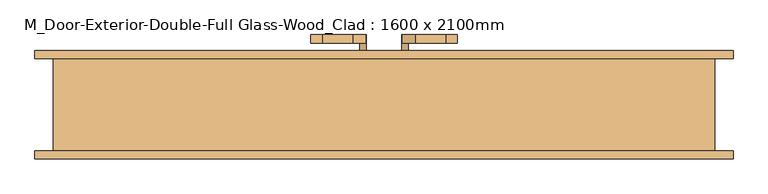
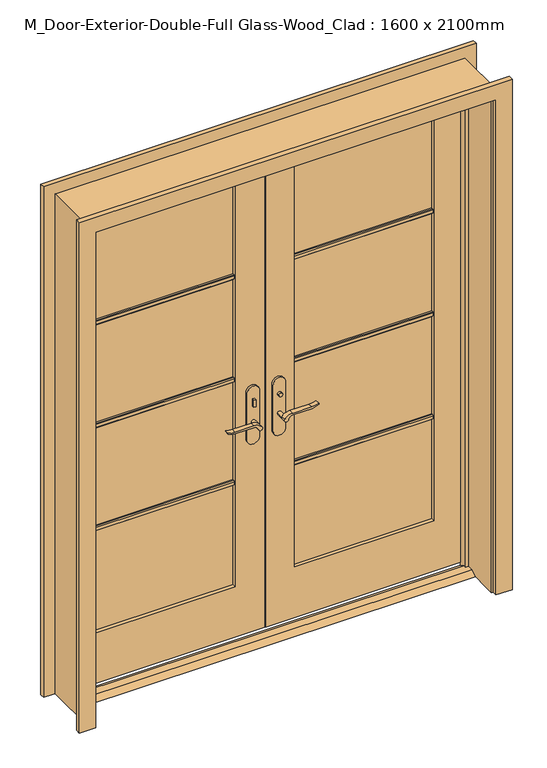
"""IFC4 building model written with IfcOpenShell, lengths in millimetres: door geometry, M_Door-Exterior-Double-Full Glass-Wood_Clad : 1600 x 2100mm."""

import ifcopenshell
import ifcopenshell.guid

model = None  # the IFC model being written
_history = None  # IfcOwnerHistory: only IFC2X3 demands one
_inside = {}  # id of a spatial element -> (the spatial element, [elements in it])
_under = {}  # id of a project, library or spatial element -> (it, [spatial elements below it])
_declared = {}  # id of a project -> (the project, [libraries it declares])
_typed = {}  # id of a type object -> (the type object, [elements of that type])
_made_of = {}  # id of a material, layer set ... -> (it, [elements and type objects made of it])


def new_model(schema):
    """Start an empty IFC model of exactly this schema.

    Asked for "IFC4X3", IfcOpenShell would pick the latest addendum, in which some entities
    have other attributes; the version numbers below select the first issue.
    IFC2X3 requires an IfcOwnerHistory on every rooted entity: one is made here for all.
    """
    global model, _history
    if schema == "IFC4X3":
        model = ifcopenshell.file(schema_version=(4, 3, 0, 0))
    else:
        model = ifcopenshell.file(schema=schema)
    _inside.clear()
    _under.clear()
    _declared.clear()
    _typed.clear()
    _made_of.clear()
    _history = None
    if model.schema == "IFC2X3":
        org = make("IfcOrganization", Name="unknown")
        user = make(
            "IfcPersonAndOrganization",
            ThePerson=make("IfcPerson", FamilyName="unknown"),
            TheOrganization=org,
        )
        app = make(
            "IfcApplication",
            ApplicationDeveloper=org,
            Version="unknown",
            ApplicationFullName="unknown",
            ApplicationIdentifier="unknown",
        )
        _history = make(
            "IfcOwnerHistory",
            OwningUser=user,
            OwningApplication=app,
            ChangeAction="ADDED",
            CreationDate=0,
        )
    return model


def make(cls, **values):
    """One entity of the class cls with the attributes given. An attribute that is None is left unset."""
    return model.create_entity(
        cls, **{name: value for name, value in values.items() if value is not None}
    )


def rooted(cls, **values):
    """An entity with a GlobalId (a new one), such as an element, a storey or a relation."""
    return make(cls, GlobalId=ifcopenshell.guid.new(), OwnerHistory=_history, **values)


def si_unit(unit_type, name, prefix=None):
    """IfcSIUnit, for example si_unit("LENGTHUNIT", "METRE", prefix="MILLI")."""
    return make("IfcSIUnit", UnitType=unit_type, Prefix=prefix, Name=name)


def assignment(units):
    """IfcUnitAssignment: the units of a project."""
    return None if units is None else make("IfcUnitAssignment", Units=units)


def point(xyz):
    """IfcCartesianPoint."""
    return None if xyz is None else make("IfcCartesianPoint", Coordinates=xyz)


def direction(xyz):
    """IfcDirection."""
    return None if xyz is None else make("IfcDirection", DirectionRatios=xyz)


def frame(location, z_axis=None, x_axis=None):
    """IfcAxis2Placement3D, a coordinate frame: its origin and axes. An axis left out is left unset."""
    return make(
        "IfcAxis2Placement3D",
        Location=point(location),
        Axis=direction(z_axis),
        RefDirection=direction(x_axis),
    )


def frame_2d(location, x_axis=None):
    """IfcAxis2Placement2D, a coordinate frame in the plane: its origin and x axis."""
    return make(
        "IfcAxis2Placement2D", Location=point(location), RefDirection=direction(x_axis)
    )


def origin():
    """The frame at (0, 0, 0) with its axes left unset."""
    return frame((0.0, 0.0, 0.0))


def place(relative_to, where):
    """IfcLocalPlacement: puts the frame where relative to a parent placement (None: the world)."""
    return make(
        "IfcLocalPlacement", PlacementRelTo=relative_to, RelativePlacement=where
    )


def context(
    kind, dimensions, precision=None, world=None, true_north=None, identifier=None
):
    """IfcGeometricRepresentationContext, for example the 3D "Model" context."""
    return make(
        "IfcGeometricRepresentationContext",
        ContextIdentifier=identifier,
        ContextType=kind,
        CoordinateSpaceDimension=dimensions,
        Precision=precision,
        WorldCoordinateSystem=world,
        TrueNorth=true_north,
    )


def project(units=None, contexts=None):
    """IfcProject with its units and contexts."""
    return rooted(
        "IfcProject",
        Name="project",
        RepresentationContexts=contexts,
        UnitsInContext=assignment(units),
    )


def spatial(cls, under=None, at=None, **own):
    """A site, building, storey or space (cls), placed at a placement, below another one or the project."""
    s = rooted(cls, ObjectPlacement=at, **own)
    if under is not None:
        _under.setdefault(under.id(), (under, []))[1].append(s)
    return s


def polyline(points):
    """IfcPolyline through the points."""
    return make("IfcPolyline", Points=[point(p) for p in points])


def circle_curve(where, radius):
    """IfcCircle in the frame where."""
    return make("IfcCircle", Position=where, Radius=radius)


def trimmed(basis, trim1, trim2, sense, master):
    """IfcTrimmedCurve: the piece of a basis curve between two trims."""
    return make(
        "IfcTrimmedCurve",
        BasisCurve=basis,
        Trim1=trim1,
        Trim2=trim2,
        SenseAgreement=sense,
        MasterRepresentation=master,
    )


def segment(curve, same_sense, transition):
    """IfcCompositeCurveSegment."""
    return make(
        "IfcCompositeCurveSegment",
        Transition=transition,
        SameSense=same_sense,
        ParentCurve=curve,
    )


def composite_curve(segments, self_intersect=None):
    """IfcCompositeCurve: segments joined end to end."""
    return make("IfcCompositeCurve", Segments=segments, SelfIntersect=self_intersect)


def outline(outer, holes=None, kind="AREA"):
    """IfcArbitraryClosedProfileDef: a profile drawn as a closed curve; with holes, ...WithVoids."""
    if holes is None:
        return make("IfcArbitraryClosedProfileDef", ProfileType=kind, OuterCurve=outer)
    return make(
        "IfcArbitraryProfileDefWithVoids",
        ProfileType=kind,
        OuterCurve=outer,
        InnerCurves=holes,
    )


def extrude(swept, where, along, depth):
    """IfcExtrudedAreaSolid: the profile swept, set in the frame where, extruded along a direction by depth."""
    return make(
        "IfcExtrudedAreaSolid",
        SweptArea=swept,
        Position=where,
        ExtrudedDirection=direction(along),
        Depth=depth,
    )


def faces_of(points, faces, orient=None, outer=None):
    """IfcFace entities. A face is a list of loops; a loop is a list of indices into points, from 0.

    orient and outer hold one flag for each loop. By default every Orientation is true, the
    first loop of a face is its IfcFaceOuterBound and the others are IfcFaceBound.
    """
    made = []
    for i, loops in enumerate(faces):
        bounds = []
        for j, loop in enumerate(loops):
            is_outer = j == 0 if outer is None else outer[i][j]
            bounds.append(
                make(
                    "IfcFaceOuterBound" if is_outer else "IfcFaceBound",
                    Bound=make("IfcPolyLoop", Polygon=[points[k] for k in loop]),
                    Orientation=True if orient is None else orient[i][j],
                )
            )
        made.append(make("IfcFace", Bounds=bounds))
    return made


def faceted_brep(points, faces, orient=None, outer=None, voids=None):
    """IfcFacetedBrep: a solid bounded by flat faces; with voids (closed shells), ...WithVoids."""
    shared = [point(p) for p in points]
    hull = make("IfcClosedShell", CfsFaces=faces_of(shared, faces, orient, outer))
    if voids is None:
        return make("IfcFacetedBrep", Outer=hull)
    return make(
        "IfcFacetedBrepWithVoids",
        Outer=hull,
        Voids=[
            make(cls, CfsFaces=faces_of(shared, fs, o, b)) for cls, fs, o, b in voids
        ],
    )


def shape(context_of_items, identifier, shape_type, items):
    """IfcShapeRepresentation: the items that make up one representation, for example the "Body"."""
    return make(
        "IfcShapeRepresentation",
        ContextOfItems=context_of_items,
        RepresentationIdentifier=identifier,
        RepresentationType=shape_type,
        Items=items,
    )


def source(mapping_origin, context_of_items, identifier, shape_type, items):
    """IfcRepresentationMap: a shape defined once, which mapped items show again and again."""
    return make(
        "IfcRepresentationMap",
        MappingOrigin=mapping_origin,
        MappedRepresentation=shape(context_of_items, identifier, shape_type, items),
    )


def transform(
    local_origin,
    x_axis=None,
    y_axis=None,
    z_axis=None,
    scale=None,
    scale2=None,
    scale3=None,
    uniform=True,
):
    """IfcCartesianTransformationOperator3D, or its non-uniform kind. x_axis, y_axis, z_axis: its Axis1, 2, 3."""
    if uniform:
        return make(
            "IfcCartesianTransformationOperator3D",
            Axis1=direction(x_axis),
            Axis2=direction(y_axis),
            LocalOrigin=point(local_origin),
            Scale=scale,
            Axis3=direction(z_axis),
        )
    return make(
        "IfcCartesianTransformationOperator3DnonUniform",
        Axis1=direction(x_axis),
        Axis2=direction(y_axis),
        LocalOrigin=point(local_origin),
        Scale=scale,
        Axis3=direction(z_axis),
        Scale2=scale2,
        Scale3=scale3,
    )


def mapped(mapping_source, mapping_target):
    """IfcMappedItem: shows the shape of a source again, moved by a transform."""
    return make(
        "IfcMappedItem", MappingSource=mapping_source, MappingTarget=mapping_target
    )


def made_of(thing, what):
    """Note that an element or type object is made of a material, layer set ...; save() writes the relation."""
    if what is not None:
        _made_of.setdefault(what.id(), (what, []))[1].append(thing)
    return thing


def element(
    cls,
    number,
    at=None,
    inside=None,
    cuts=None,
    type_object=None,
    material=None,
    context=None,
    identifier="Body",
    shape_type=None,
    held_by="IfcProductDefinitionShape",
    body=None,
    shapes=None,
    **own,
):
    """One element of the class cls, such as IfcWall. Its Tag is "e" and its number.

    at: its placement. inside: the storey or other place that contains it. cuts: it is an
    opening in that element (IfcRelVoidsElement). A single representation is given by context,
    identifier, shape_type and body (its items); several are given by shapes. held_by: the class
    of the entity that holds the representations. save() writes the other relations.
    """
    e = rooted(cls, Tag="e%d" % number, ObjectPlacement=at, **own)
    if body is not None:
        shapes = [shape(context, identifier, shape_type, body)]
    if shapes is not None:
        e.Representation = make(held_by, Representations=shapes)
    if inside is not None:
        _inside.setdefault(inside.id(), (inside, []))[1].append(e)
    if cuts is not None:
        rooted(
            "IfcRelVoidsElement", RelatingBuildingElement=cuts, RelatedOpeningElement=e
        )
    if type_object is not None:
        _typed.setdefault(type_object.id(), (type_object, []))[1].append(e)
    return made_of(e, material)


def aggregate(whole, parts):
    """IfcRelAggregates: a whole, such as a stair, and the parts it consists of."""
    return rooted("IfcRelAggregates", RelatingObject=whole, RelatedObjects=parts)


def save(model, path):
    """Write the relations noted so far, then the file.

    IfcRelAggregates (storeys below a building ...), IfcRelContainedInSpatialStructure (elements
    in a storey), IfcRelDefinesByType, IfcRelAssociatesMaterial and IfcRelDeclares: one each for
    every whole, place, type object, material and project.
    """
    for whole, parts in _under.values():
        aggregate(whole, parts)
    for where, things in _inside.values():
        rooted(
            "IfcRelContainedInSpatialStructure",
            RelatedElements=things,
            RelatingStructure=where,
        )
    for kind, things in _typed.values():
        rooted("IfcRelDefinesByType", RelatedObjects=things, RelatingType=kind)
    for what, things in _made_of.values():
        rooted("IfcRelAssociatesMaterial", RelatedObjects=things, RelatingMaterial=what)
    for by, libraries in _declared.values():
        rooted("IfcRelDeclares", RelatingContext=by, RelatedDefinitions=libraries)
    model.write(path)


def m_door_exterior_double_full_glass_wood_clad_1600_x_2100mm_56e3e291(model_context):
    return source(origin(), model_context, "Body", "SolidModel", [
        extrude(outline(polyline([(18.975, 15.0), (53.975, 15.0), (79.375, 0.0), (-6.425, 0.0), (18.975, 15.0)])), frame((-800.0, 0.0, 0.0), z_axis=(1.0, 0.0, 0.0), x_axis=(0.0, 1.0, 0.0)), (0.0, 0.0, 1.0), 1600.0),
        extrude(outline(polyline([(-47.4019111, 56.825), (-57.4019111, 56.825), (-57.4019111, 66.825), (-47.4019111, 66.825), (-47.4019111, 56.825)])), frame((0.0, 0.0, 981.9), z_axis=(0.0, 0.0, 1.0), x_axis=(1.0, 0.0, 0.0)), (0.0, 0.0, 1.0), 30.0),
        extrude(outline(composite_curve([segment(trimmed(circle_curve(frame_2d((996.9, -52.4019111)), 8.0), [point((996.9, -60.4019111))], [point((996.9, -44.4019111))], False, "CARTESIAN"), True, "CONTINUOUS"), segment(trimmed(circle_curve(frame_2d((996.9, -52.4019111)), 8.0), [point((996.9, -44.4019111))], [point((996.9, -60.4019111))], False, "CARTESIAN"), True, "CONTINUOUS")], self_intersect=False)), frame((0.0, 121.825, 0.0), z_axis=(0.0, 1.0, 0.0), x_axis=(0.0, 0.0, 1.0)), (0.0, 0.0, 1.0), 10.0),
        extrude(outline(composite_curve([segment(trimmed(circle_curve(frame_2d((897.1555521, -76.0694241)), 37.2832219), [point((919.0523287, -45.8937749))], [point((934.4, -77.7693445))], False, "CARTESIAN"), True, "CONTINUOUS"), segment(polyline([(934.4, -77.7693445), (934.4, -154.045502)]), True, "CONTINUOUS"), segment(trimmed(circle_curve(frame_2d((1017.6850638, -153.9791202)), 83.2850902), [point((934.4, -154.045502))], [point((939.4, -182.4019111))], True, "CARTESIAN"), True, "CONTINUOUS"), segment(polyline([(939.4, -182.4019111), (936.6135558, -182.4019111)]), True, "CONTINUOUS"), segment(trimmed(circle_curve(frame_2d((986.6709207, -150.4622499)), 59.3791355), [point((936.6135558, -182.4019111))], [point((927.4, -154.045502))], False, "CARTESIAN"), True, "CONTINUOUS"), segment(polyline([(927.4, -154.045502), (927.4, -77.7881013)]), True, "CONTINUOUS"), segment(trimmed(circle_curve(frame_2d((909.2738613, -77.7881013)), 18.1261387), [point((927.4, -77.7881013))], [point((914.4, -60.4019111))], True, "CARTESIAN"), True, "CONTINUOUS"), segment(trimmed(circle_curve(frame_2d((914.4, -52.4019111)), 8.0), [point((914.4, -60.4019111))], [point((919.0523287, -45.8937749))], False, "CARTESIAN"), True, "CONTINUOUS")], self_intersect=False)), frame((0.0, 16.825, 0.0), z_axis=(0.0, 1.0, 0.0), x_axis=(0.0, 0.0, 1.0)), (0.0, 0.0, 1.0), 20.0),
        extrude(outline(composite_curve([segment(trimmed(circle_curve(frame_2d((914.4, -52.4019111)), 8.0), [point((914.3999903, -60.4019111))], [point((919.0523287, -45.8937749))], False, "CARTESIAN"), True, "CONTINUOUS"), segment(trimmed(circle_curve(frame_2d((897.1555521, -76.0694241)), 37.2832219), [point((919.0523287, -45.8937749))], [point((934.4, -77.7693445))], False, "CARTESIAN"), True, "CONTINUOUS"), segment(polyline([(934.4, -77.7693445), (934.4, -154.045502)]), True, "CONTINUOUS"), segment(trimmed(circle_curve(frame_2d((1017.6850638, -153.9791202)), 83.2850902), [point((934.4, -154.045502))], [point((939.4, -182.4019111))], True, "CARTESIAN"), True, "CONTINUOUS"), segment(polyline([(939.4, -182.4019111), (936.6135558, -182.4019111)]), True, "CONTINUOUS"), segment(trimmed(circle_curve(frame_2d((986.6709207, -150.4622499)), 59.3791355), [point((936.6135558, -182.4019111))], [point((927.4, -154.045502))], False, "CARTESIAN"), True, "CONTINUOUS"), segment(polyline([(927.4, -154.045502), (927.4, -77.788099)]), True, "CONTINUOUS"), segment(trimmed(circle_curve(frame_2d((909.2738682, -77.788099)), 18.1261318), [point((927.4, -77.788099))], [point((914.3999903, -60.4019111))], True, "CARTESIAN"), True, "CONTINUOUS")], self_intersect=False)), frame((0.0, 151.825, 0.0), z_axis=(0.0, 1.0, 0.0), x_axis=(0.0, 0.0, 1.0)), (0.0, 0.0, 1.0), 20.0),
        extrude(outline(composite_curve([segment(trimmed(circle_curve(frame_2d((914.4, -52.4019111)), 8.0), [point((914.4, -60.4019111))], [point((914.4, -44.4019111))], False, "CARTESIAN"), True, "CONTINUOUS"), segment(trimmed(circle_curve(frame_2d((914.4, -52.4019111)), 8.0), [point((914.4, -44.4019111))], [point((914.4, -60.4019111))], False, "CARTESIAN"), True, "CONTINUOUS")], self_intersect=False)), frame((0.0, 36.825, 0.0), z_axis=(0.0, 1.0, 0.0), x_axis=(0.0, 0.0, 1.0)), (0.0, 0.0, 1.0), 30.0),
        extrude(outline(composite_curve([segment(trimmed(circle_curve(frame_2d((914.4, -52.4019111)), 8.0), [point((914.4, -60.4019111))], [point((914.4, -44.4019111))], False, "CARTESIAN"), True, "CONTINUOUS"), segment(trimmed(circle_curve(frame_2d((914.4, -52.4019111)), 8.0), [point((914.4, -44.4019111))], [point((914.4, -60.4019111))], False, "CARTESIAN"), True, "CONTINUOUS")], self_intersect=False)), frame((0.0, 121.825, 0.0), z_axis=(0.0, 1.0, 0.0), x_axis=(0.0, 0.0, 1.0)), (0.0, 0.0, 1.0), 30.0),
        extrude(outline(composite_curve([segment(polyline([(844.4, -27.4019111), (1039.4, -27.4019111)]), True, "CONTINUOUS"), segment(trimmed(circle_curve(frame_2d((1039.4, -52.4019111)), 25.0), [point((1039.4, -27.4019111))], [point((1039.4, -77.4019111))], False, "CARTESIAN"), True, "CONTINUOUS"), segment(polyline([(1039.4, -77.4019111), (844.4, -77.4019111)]), True, "CONTINUOUS"), segment(trimmed(circle_curve(frame_2d((844.4, -52.4019111)), 25.0), [point((844.4, -77.4019111))], [point((844.4, -27.4019111))], False, "CARTESIAN"), True, "CONTINUOUS")], self_intersect=False)), frame((0.0, 66.825, 0.0), z_axis=(0.0, 1.0, 0.0), x_axis=(0.0, 0.0, 1.0)), (0.0, 0.0, 1.0), 10.0),
        extrude(outline(composite_curve([segment(polyline([(844.4, -27.4019111), (1039.4, -27.4019111)]), True, "CONTINUOUS"), segment(trimmed(circle_curve(frame_2d((1039.4, -52.4019111)), 25.0), [point((1039.4, -27.4019111))], [point((1039.4, -77.4019111))], False, "CARTESIAN"), True, "CONTINUOUS"), segment(polyline([(1039.4, -77.4019111), (844.4, -77.4019111)]), True, "CONTINUOUS"), segment(trimmed(circle_curve(frame_2d((844.4, -52.4019111)), 25.0), [point((844.4, -77.4019111))], [point((844.4, -27.4019111))], False, "CARTESIAN"), True, "CONTINUOUS")], self_intersect=False)), frame((0.0, 111.825, 0.0), z_axis=(0.0, 1.0, 0.0), x_axis=(0.0, 0.0, 1.0)), (0.0, 0.0, 1.0), 10.0),
        extrude(outline(polyline([(47.3875, 131.825), (57.3875, 131.825), (57.3875, 121.825), (47.3875, 121.825), (47.3875, 131.825)])), frame((0.0, 0.0, 981.9), z_axis=(0.0, 0.0, 1.0), x_axis=(1.0, 0.0, 0.0)), (0.0, 0.0, 1.0), 30.0),
        extrude(outline(composite_curve([segment(trimmed(circle_curve(frame_2d((996.9, 52.3875)), 8.0), [point((996.9, 60.3875))], [point((996.9, 44.3875))], False, "CARTESIAN"), True, "CONTINUOUS"), segment(trimmed(circle_curve(frame_2d((996.9, 52.3875)), 8.0), [point((996.9, 44.3875))], [point((996.9, 60.3875))], False, "CARTESIAN"), True, "CONTINUOUS")], self_intersect=False)), frame((0.0, 56.825, 0.0), z_axis=(0.0, 1.0, 0.0), x_axis=(0.0, 0.0, 1.0)), (0.0, 0.0, 1.0), 10.0),
        extrude(outline(composite_curve([segment(trimmed(circle_curve(frame_2d((914.4, 52.3875)), 8.0), [point((919.0523287, 45.8793637))], [point((914.4, 60.3875))], False, "CARTESIAN"), True, "CONTINUOUS"), segment(trimmed(circle_curve(frame_2d((909.2738613, 77.7736901)), 18.1261387), [point((914.4, 60.3875))], [point((927.4, 77.7736901))], True, "CARTESIAN"), True, "CONTINUOUS"), segment(polyline([(927.4, 77.7736901), (927.4, 154.0310909)]), True, "CONTINUOUS"), segment(trimmed(circle_curve(frame_2d((986.6709207, 150.4478388)), 59.3791355), [point((927.4, 154.0310909))], [point((936.6135558, 182.3875))], False, "CARTESIAN"), True, "CONTINUOUS"), segment(polyline([(936.6135558, 182.3875), (939.4, 182.3875)]), True, "CONTINUOUS"), segment(trimmed(circle_curve(frame_2d((1017.6850638, 153.9647091)), 83.2850902), [point((939.4, 182.3875))], [point((934.4, 154.0310909))], True, "CARTESIAN"), True, "CONTINUOUS"), segment(polyline([(934.4, 154.0310909), (934.4, 77.7549333)]), True, "CONTINUOUS"), segment(trimmed(circle_curve(frame_2d((897.1555521, 76.0550129)), 37.2832219), [point((934.4, 77.7549333))], [point((919.0523287, 45.8793637))], False, "CARTESIAN"), True, "CONTINUOUS")], self_intersect=False)), frame((0.0, 151.825, 0.0), z_axis=(0.0, 1.0, 0.0), x_axis=(0.0, 0.0, 1.0)), (0.0, 0.0, 1.0), 20.0),
        extrude(outline(composite_curve([segment(trimmed(circle_curve(frame_2d((909.2738682, 77.7736878)), 18.1261318), [point((914.3999903, 60.3875))], [point((927.4, 77.7736878))], True, "CARTESIAN"), True, "CONTINUOUS"), segment(polyline([(927.4, 77.7736878), (927.4, 154.0310909)]), True, "CONTINUOUS"), segment(trimmed(circle_curve(frame_2d((986.6709207, 150.4478388)), 59.3791355), [point((927.4, 154.0310909))], [point((936.6135558, 182.3875))], False, "CARTESIAN"), True, "CONTINUOUS"), segment(polyline([(936.6135558, 182.3875), (939.4, 182.3875)]), True, "CONTINUOUS"), segment(trimmed(circle_curve(frame_2d((1017.6850638, 153.9647091)), 83.2850902), [point((939.4, 182.3875))], [point((934.4, 154.0310909))], True, "CARTESIAN"), True, "CONTINUOUS"), segment(polyline([(934.4, 154.0310909), (934.4, 77.7549333)]), True, "CONTINUOUS"), segment(trimmed(circle_curve(frame_2d((897.1555521, 76.0550129)), 37.2832219), [point((934.4, 77.7549333))], [point((919.0523287, 45.8793637))], False, "CARTESIAN"), True, "CONTINUOUS"), segment(trimmed(circle_curve(frame_2d((914.4, 52.3875)), 8.0), [point((919.0523287, 45.8793637))], [point((914.3999903, 60.3875))], False, "CARTESIAN"), True, "CONTINUOUS")], self_intersect=False)), frame((0.0, 16.825, 0.0), z_axis=(0.0, 1.0, 0.0), x_axis=(0.0, 0.0, 1.0)), (0.0, 0.0, 1.0), 20.0),
        extrude(outline(composite_curve([segment(trimmed(circle_curve(frame_2d((914.4, 52.3875)), 8.0), [point((914.4, 60.3875))], [point((914.4, 44.3875))], False, "CARTESIAN"), True, "CONTINUOUS"), segment(trimmed(circle_curve(frame_2d((914.4, 52.3875)), 8.0), [point((914.4, 44.3875))], [point((914.4, 60.3875))], False, "CARTESIAN"), True, "CONTINUOUS")], self_intersect=False)), frame((0.0, 121.825, 0.0), z_axis=(0.0, 1.0, 0.0), x_axis=(0.0, 0.0, 1.0)), (0.0, 0.0, 1.0), 30.0),
        extrude(outline(composite_curve([segment(trimmed(circle_curve(frame_2d((914.4, 52.3875)), 8.0), [point((914.4, 60.3875))], [point((914.4, 44.3875))], False, "CARTESIAN"), True, "CONTINUOUS"), segment(trimmed(circle_curve(frame_2d((914.4, 52.3875)), 8.0), [point((914.4, 44.3875))], [point((914.4, 60.3875))], False, "CARTESIAN"), True, "CONTINUOUS")], self_intersect=False)), frame((0.0, 36.825, 0.0), z_axis=(0.0, 1.0, 0.0), x_axis=(0.0, 0.0, 1.0)), (0.0, 0.0, 1.0), 30.0),
        extrude(outline(composite_curve([segment(trimmed(circle_curve(frame_2d((844.4, 52.3875)), 25.0), [point((844.4, 27.3875))], [point((844.4, 77.3875))], False, "CARTESIAN"), True, "CONTINUOUS"), segment(polyline([(844.4, 77.3875), (1039.4, 77.3875)]), True, "CONTINUOUS"), segment(trimmed(circle_curve(frame_2d((1039.4, 52.3875)), 25.0), [point((1039.4, 77.3875))], [point((1039.4, 27.3875))], False, "CARTESIAN"), True, "CONTINUOUS"), segment(polyline([(1039.4, 27.3875), (844.4, 27.3875)]), True, "CONTINUOUS")], self_intersect=False)), frame((0.0, 111.825, 0.0), z_axis=(0.0, 1.0, 0.0), x_axis=(0.0, 0.0, 1.0)), (0.0, 0.0, 1.0), 10.0),
        extrude(outline(composite_curve([segment(trimmed(circle_curve(frame_2d((844.4, 52.3875)), 25.0), [point((844.4, 27.3875))], [point((844.4, 77.3875))], False, "CARTESIAN"), True, "CONTINUOUS"), segment(polyline([(844.4, 77.3875), (1039.4, 77.3875)]), True, "CONTINUOUS"), segment(trimmed(circle_curve(frame_2d((1039.4, 52.3875)), 25.0), [point((1039.4, 77.3875))], [point((1039.4, 27.3875))], False, "CARTESIAN"), True, "CONTINUOUS"), segment(polyline([(1039.4, 27.3875), (844.4, 27.3875)]), True, "CONTINUOUS")], self_intersect=False)), frame((0.0, 66.825, 0.0), z_axis=(0.0, 1.0, 0.0), x_axis=(0.0, 0.0, 1.0)), (0.0, 0.0, 1.0), 10.0),
        extrude(outline(polyline([(90.825, 1552.025), (90.825, 1532.975), (84.475, 1532.975), (81.3, 1536.15), (81.3, 1548.85), (84.475, 1552.025), (90.825, 1552.025)])), frame((120.0, 0.0, 0.0), z_axis=(1.0, 0.0, 0.0), x_axis=(0.0, 1.0, 0.0)), (0.0, 0.0, 1.0), 560.0),
        extrude(outline(polyline([(90.825, 1114.525), (90.825, 1095.475), (84.475, 1095.475), (81.3, 1098.65), (81.3, 1111.35), (84.475, 1114.525), (90.825, 1114.525)])), frame((120.0, 0.0, 0.0), z_axis=(1.0, 0.0, 0.0), x_axis=(0.0, 1.0, 0.0)), (0.0, 0.0, 1.0), 560.0),
        extrude(outline(polyline([(90.825, 677.025), (90.825, 657.975), (84.475, 657.975), (81.3, 661.15), (81.3, 673.85), (84.475, 677.025), (90.825, 677.025)])), frame((120.0, 0.0, 0.0), z_axis=(1.0, 0.0, 0.0), x_axis=(0.0, 1.0, 0.0)), (0.0, 0.0, 1.0), 560.0),
        extrude(outline(polyline([(97.825, 1552.025), (104.175, 1552.025), (107.35, 1548.85), (107.35, 1536.15), (104.175, 1532.975), (97.825, 1532.975), (97.825, 1552.025)])), frame((-680.0, 0.0, 0.0), z_axis=(1.0, 0.0, 0.0), x_axis=(0.0, 1.0, 0.0)), (0.0, 0.0, 1.0), 560.0),
        extrude(outline(polyline([(97.825, 1114.525), (104.175, 1114.525), (107.35, 1111.35), (107.35, 1098.65), (104.175, 1095.475), (97.825, 1095.475), (97.825, 1114.525)])), frame((-680.0, 0.0, 0.0), z_axis=(1.0, 0.0, 0.0), x_axis=(0.0, 1.0, 0.0)), (0.0, 0.0, 1.0), 560.0),
        extrude(outline(polyline([(97.825, 677.025), (104.175, 677.025), (107.35, 673.85), (107.35, 661.15), (104.175, 657.975), (97.825, 657.975), (97.825, 677.025)])), frame((-680.0, 0.0, 0.0), z_axis=(1.0, 0.0, 0.0), x_axis=(0.0, 1.0, 0.0)), (0.0, 0.0, 1.0), 560.0),
        extrude(outline(polyline([(97.825, 1552.025), (104.175, 1552.025), (107.35, 1548.85), (107.35, 1536.15), (104.175, 1532.975), (97.825, 1532.975), (97.825, 1552.025)])), frame((120.0, 0.0, 0.0), z_axis=(1.0, 0.0, 0.0), x_axis=(0.0, 1.0, 0.0)), (0.0, 0.0, 1.0), 560.0),
        extrude(outline(polyline([(97.825, 1114.525), (104.175, 1114.525), (107.35, 1111.35), (107.35, 1098.65), (104.175, 1095.475), (97.825, 1095.475), (97.825, 1114.525)])), frame((120.0, 0.0, 0.0), z_axis=(1.0, 0.0, 0.0), x_axis=(0.0, 1.0, 0.0)), (0.0, 0.0, 1.0), 560.0),
        extrude(outline(polyline([(97.825, 677.025), (104.175, 677.025), (107.35, 673.85), (107.35, 661.15), (104.175, 657.975), (97.825, 657.975), (97.825, 677.025)])), frame((120.0, 0.0, 0.0), z_axis=(1.0, 0.0, 0.0), x_axis=(0.0, 1.0, 0.0)), (0.0, 0.0, 1.0), 560.0),
        extrude(outline(polyline([(90.825, 1552.025), (90.825, 1532.975), (84.475, 1532.975), (81.3, 1536.15), (81.3, 1548.85), (84.475, 1552.025), (90.825, 1552.025)])), frame((-680.0, 0.0, 0.0), z_axis=(1.0, 0.0, 0.0), x_axis=(0.0, 1.0, 0.0)), (0.0, 0.0, 1.0), 560.0),
        extrude(outline(polyline([(90.825, 1114.525), (90.825, 1095.475), (84.475, 1095.475), (81.3, 1098.65), (81.3, 1111.35), (84.475, 1114.525), (90.825, 1114.525)])), frame((-680.0, 0.0, 0.0), z_axis=(1.0, 0.0, 0.0), x_axis=(0.0, 1.0, 0.0)), (0.0, 0.0, 1.0), 560.0),
        extrude(outline(polyline([(90.825, 677.025), (90.825, 657.975), (84.475, 657.975), (81.3, 661.15), (81.3, 673.85), (84.475, 677.025), (90.825, 677.025)])), frame((-680.0, 0.0, 0.0), z_axis=(1.0, 0.0, 0.0), x_axis=(0.0, 1.0, 0.0)), (0.0, 0.0, 1.0), 560.0),
        extrude(outline(polyline([(0.0, 806.35), (0.0, 871.35), (2171.35, 871.35), (2171.35, -871.35), (0.0, -871.35), (0.0, -806.35), (2106.35, -806.35), (2106.35, 806.35), (0.0, 806.35)])), frame((0.0, 111.825, 0.0), z_axis=(0.0, 1.0, 0.0), x_axis=(0.0, 0.0, 1.0)), (0.0, 0.0, 1.0), 20.0),
        extrude(outline(polyline([(0.0, 806.35), (0.0, 871.35), (2171.35, 871.35), (2171.35, -871.35), (0.0, -871.35), (0.0, -806.35), (2106.35, -806.35), (2106.35, 806.35), (0.0, 806.35)])), frame((0.0, -138.175, 0.0), z_axis=(0.0, 1.0, 0.0), x_axis=(0.0, 0.0, 1.0)), (0.0, 0.0, 1.0), 20.0),
        extrude(outline(polyline([(15.0, 800.0), (2100.0, 800.0), (2100.0, 1.5875), (15.0, 1.5875), (15.0, 800.0)]), holes=[polyline([(1980.0, 120.0), (1980.0, 680.0), (230.0, 680.0), (230.0, 120.0), (1980.0, 120.0)])]), frame((0.0, 76.825, 0.0), z_axis=(0.0, 1.0, 0.0), x_axis=(0.0, 0.0, 1.0)), (0.0, 0.0, 1.0), 35.0),
        extrude(outline(polyline([(2100.0, -800.0), (15.0, -800.0), (15.0, -1.6019111), (2100.0, -1.6019111), (2100.0, -800.0)]), holes=[polyline([(230.0, -680.0), (1980.0, -680.0), (1980.0, -120.0), (230.0, -120.0), (230.0, -680.0)])]), frame((0.0, 76.825, 0.0), z_axis=(0.0, 1.0, 0.0), x_axis=(0.0, 0.0, 1.0)), (0.0, 0.0, 1.0), 35.0),
        faceted_brep([(825.0, 111.825, 0.0), (825.0, -118.175, 0.0), (800.0, -118.175, 0.0), (800.0, 41.9, 0.0), (787.3, 41.9, 0.0), (787.3, 76.825, 0.0), (800.0, 76.825, 0.0), (800.0, 111.825, 0.0), (825.0, 111.825, 2125.0), (825.0, -118.175, 2125.0), (-825.0, -118.175, 2125.0), (-825.0, -118.175, 0.0), (-800.0, -118.175, 0.0), (-800.0, -118.175, 2100.0), (800.0, -118.175, 2100.0), (800.0, 41.9, 2100.0), (-800.0, 41.9, 2100.0), (-800.0, 41.9, 0.0), (-787.3, 41.9, 0.0), (-787.3, 41.9, 2087.3), (787.3, 41.9, 2087.3), (787.3, 76.825, 2087.3), (1.5875, 76.825, 2087.3), (-1.6019111, 76.825, 2087.3), (-787.3, 76.825, 2087.3), (-787.3, 76.825, 0.0), (-800.0, 76.825, 0.0), (-800.0, 76.825, 2100.0), (-1.6019111, 76.825, 2100.0), (1.5875, 76.825, 2100.0), (800.0, 76.825, 2100.0), (800.0, 111.825, 2100.0), (1.5875, 111.825, 2100.0), (-1.6019111, 111.825, 2100.0), (-800.0, 111.825, 2100.0), (-800.0, 111.825, 0.0), (-825.0, 111.825, 0.0), (-825.0, 111.825, 2125.0)], [[[0, 1, 2, 3, 4, 5, 6, 7]], [[1, 0, 8, 9]], [[2, 1, 9, 10, 11, 12, 13, 14]], [[3, 2, 14, 15]], [[4, 3, 15, 16, 17, 18, 19, 20]], [[5, 4, 20, 21]], [[6, 5, 21, 22, 23, 24, 25, 26, 27, 28, 29, 30]], [[7, 6, 30, 31]], [[0, 7, 31, 32, 33, 34, 35, 36, 37, 8]], [[9, 8, 37, 10]], [[14, 13, 16, 15]], [[20, 19, 24, 23, 22, 21]], [[31, 30, 29, 28, 27, 34, 33, 32]], [[12, 11, 36, 35, 26, 25, 18, 17]], [[11, 10, 37, 36]], [[13, 12, 17, 16]], [[19, 18, 25, 24]], [[27, 26, 35, 34]]]),
        extrude(outline(polyline([(680.0, 90.825), (120.0, 90.825), (120.0, 97.825), (680.0, 97.825), (680.0, 90.825)])), frame((0.0, 0.0, 230.0), z_axis=(0.0, 0.0, 1.0), x_axis=(1.0, 0.0, 0.0)), (0.0, 0.0, 1.0), 1750.0),
        extrude(outline(polyline([(-120.0, 90.825), (-680.0, 90.825), (-680.0, 97.825), (-120.0, 97.825), (-120.0, 90.825)])), frame((0.0, 0.0, 230.0), z_axis=(0.0, 0.0, 1.0), x_axis=(1.0, 0.0, 0.0)), (0.0, 0.0, 1.0), 1750.0),
    ])


if __name__ == "__main__":
    model = new_model("IFC4")
    model_context = context("Model", 3, world=origin())
    ifc_project = project(units=[si_unit("LENGTHUNIT", "METRE", prefix="MILLI")], contexts=[model_context])
    site = spatial("IfcSite", under=ifc_project)
    building = spatial("IfcBuilding", under=site)
    placement = place(None, origin())
    m_door_exterior_double_full_glass_wood_clad_1600_x_2100mm_shape = m_door_exterior_double_full_glass_wood_clad_1600_x_2100mm_56e3e291(model_context)
    element("IfcDoor", 1, ObjectType="M_Door-Exterior-Double-Full Glass-Wood_Clad : 1600 x 2100mm", at=placement, inside=building, context=model_context, shape_type="MappedRepresentation", body=[
        mapped(m_door_exterior_double_full_glass_wood_clad_1600_x_2100mm_shape, transform((0.0, 0.0, 0.0), x_axis=(1.0, 0.0, 0.0), y_axis=(0.0, 1.0, 0.0), z_axis=(0.0, 0.0, 1.0))),
    ])
    save(model, "model.ifc")

# Revit data of these elements
# Project information
#   Project Issue Date = "Issue Date"
#   Project Status = "Project Status"
#   Client Name = "Owner"
#   Project Address = "Enter address here"
#   Project Name = "Project Name"
#   Project Number = "0001"
# Type "M_Door-Exterior-Double-Full Glass-Wood_Clad : 1600 x 2100mm"
#   Type Mark = "41"
#   Assembly Code = "B2030100"
#   Analytic Construction = "French door, wood frame with double glass"
#   Top Rail = 12 cm
#   Threshold Offset [instance default] = 1.5 cm
#   Thickness = 3.5 cm
#   Thermal Resistance (R) = 0.337392 (m²·K)/W
#   Swing Angle [instance default] = 90.00°
#   Stiles = 12 cm
#   Rough Width = 165 cm
#   Rough Height = 212.5 cm
#   Panel Width = 80 cm
#   Door Offset [instance default] = 0 cm
#   Height = 210 cm
#   Width = 160 cm
#   Heat Transfer Coefficient (U) = 2.96405 W/(m²·K)
#   Bottom Rail = 23 cm
#   Exterior Trim [instance default] = yes
#   Threshold [instance default] = yes
#   Show Grill [instance default] = yes
#   Function = 1
#   Trim Material = Cherry
#   Threshold Material = Cherry
#   Panel Material = Cherry
#   Glazing = Glass
#   Frame Material = Cherry
#   Door Handle Material = Aluminum
#   Visual Light Transmittance = 0
#   Solar Heat Gain Coefficient = 0
#   Wall Closure = (empty or 0)
#   Construction Type = (empty or 0)
# Element 1 (IfcDoor, "M_Door-Exterior-Double-Full Glass-Wood_Clad : 1600 x 2100mm")
#   Materials on its faces: "Cherry", "Aluminum", "Glass"
# Materials
#   "Cherry": class "Wood", colour RGB 226 177 128, transparency 0, Description = "Prunus Serotina", Cost = 0
#   "Glass": class "Glass", colour RGB 0 128 192, transparency 0.9, Description = "Soda Lime Glass", Cost = 0
#   "Aluminum": class "Metal", colour RGB 247 247 247, transparency 0, Description = "Aluminum 6061", Cost = 0
